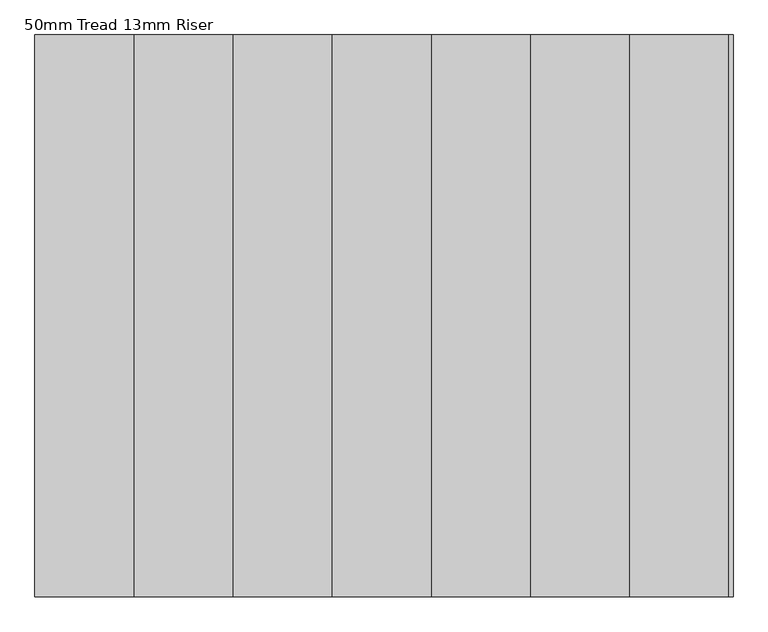
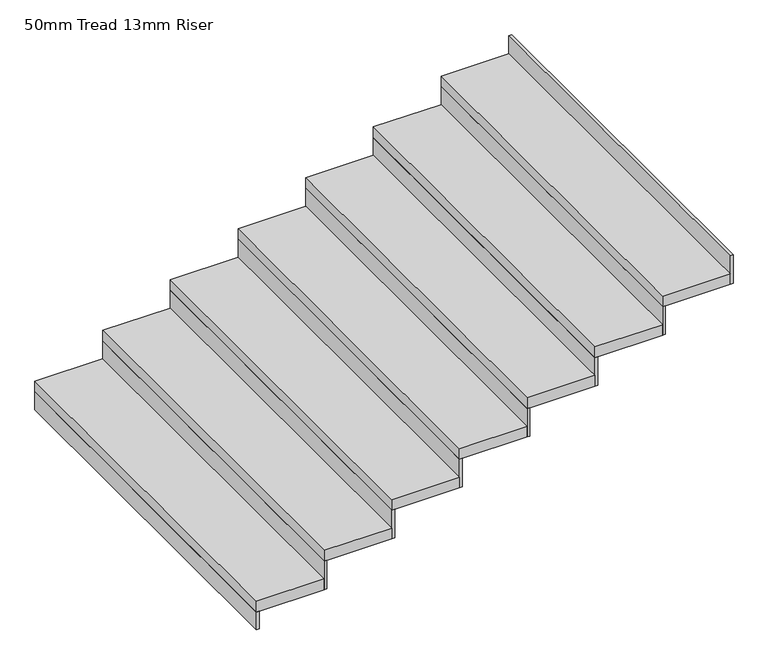
"""IFC4 building model written with IfcOpenShell, lengths in millimetres: stair flight geometry, 50mm Tread 13mm Riser."""

from ifc_helpers import new_model, si_unit, frame, origin, place, context, project, spatial, polyline, outline, extrude, source, transform, mapped, element, save


def stair_flight_50mm_tread_13mm_riser_cbb1d095(model_context):
    return source(origin(), model_context, "Body", "SweptSolid", [
        extrude(outline(polyline([(-15462.7814495, -5518.0731037), (-15475.2814495, -5518.0731037), (-15475.2814495, -3818.0731037), (-15462.7814495, -3818.0731037), (-15462.7814495, -5518.0731037)])), frame((0.0, 0.0, -2133.3333333), z_axis=(0.0, 0.0, 1.0), x_axis=(1.0, 0.0, 0.0)), (0.0, 0.0, 1.0), 83.3333333),
        extrude(outline(polyline([(-15175.2814495, -3818.0731037), (-15175.2814495, -5518.0731037), (-15475.2814495, -5518.0731037), (-15475.2814495, -3818.0731037), (-15175.2814495, -3818.0731037)])), frame((0.0, 0.0, -2050.0), z_axis=(0.0, 0.0, 1.0), x_axis=(1.0, 0.0, 0.0)), (0.0, 0.0, 1.0), 50.0),
        extrude(outline(polyline([(-15162.7814495, -5518.0731037), (-15175.2814495, -5518.0731037), (-15175.2814495, -3818.0731037), (-15162.7814495, -3818.0731037), (-15162.7814495, -5518.0731037)])), frame((0.0, 0.0, -2050.0), z_axis=(0.0, 0.0, 1.0), x_axis=(1.0, 0.0, 0.0)), (0.0, 0.0, 1.0), 133.3333333),
        extrude(outline(polyline([(-14875.2814495, -3818.0731037), (-14875.2814495, -5518.0731037), (-15175.2814495, -5518.0731037), (-15175.2814495, -3818.0731037), (-14875.2814495, -3818.0731037)])), frame((0.0, 0.0, -1916.6666667), z_axis=(0.0, 0.0, 1.0), x_axis=(1.0, 0.0, 0.0)), (0.0, 0.0, 1.0), 50.0),
        extrude(outline(polyline([(-14862.7814495, -5518.0731037), (-14875.2814495, -5518.0731037), (-14875.2814495, -3818.0731037), (-14862.7814495, -3818.0731037), (-14862.7814495, -5518.0731037)])), frame((0.0, 0.0, -1916.6666667), z_axis=(0.0, 0.0, 1.0), x_axis=(1.0, 0.0, 0.0)), (0.0, 0.0, 1.0), 133.3333333),
        extrude(outline(polyline([(-14575.2814495, -3818.0731037), (-14575.2814495, -5518.0731037), (-14875.2814495, -5518.0731037), (-14875.2814495, -3818.0731037), (-14575.2814495, -3818.0731037)])), frame((0.0, 0.0, -1783.3333333), z_axis=(0.0, 0.0, 1.0), x_axis=(1.0, 0.0, 0.0)), (0.0, 0.0, 1.0), 50.0),
        extrude(outline(polyline([(-14562.7814495, -5518.0731037), (-14575.2814495, -5518.0731037), (-14575.2814495, -3818.0731037), (-14562.7814495, -3818.0731037), (-14562.7814495, -5518.0731037)])), frame((0.0, 0.0, -1783.3333333), z_axis=(0.0, 0.0, 1.0), x_axis=(1.0, 0.0, 0.0)), (0.0, 0.0, 1.0), 133.3333333),
        extrude(outline(polyline([(-14275.2814495, -3818.0731037), (-14275.2814495, -5518.0731037), (-14575.2814495, -5518.0731037), (-14575.2814495, -3818.0731037), (-14275.2814495, -3818.0731037)])), frame((0.0, 0.0, -1650.0), z_axis=(0.0, 0.0, 1.0), x_axis=(1.0, 0.0, 0.0)), (0.0, 0.0, 1.0), 50.0),
        extrude(outline(polyline([(-14262.7814495, -5518.0731037), (-14275.2814495, -5518.0731037), (-14275.2814495, -3818.0731037), (-14262.7814495, -3818.0731037), (-14262.7814495, -5518.0731037)])), frame((0.0, 0.0, -1650.0), z_axis=(0.0, 0.0, 1.0), x_axis=(1.0, 0.0, 0.0)), (0.0, 0.0, 1.0), 133.3333333),
        extrude(outline(polyline([(-13975.2814495, -3818.0731037), (-13975.2814495, -5518.0731037), (-14275.2814495, -5518.0731037), (-14275.2814495, -3818.0731037), (-13975.2814495, -3818.0731037)])), frame((0.0, 0.0, -1516.6666667), z_axis=(0.0, 0.0, 1.0), x_axis=(1.0, 0.0, 0.0)), (0.0, 0.0, 1.0), 50.0),
        extrude(outline(polyline([(-13962.7814495, -5518.0731037), (-13975.2814495, -5518.0731037), (-13975.2814495, -3818.0731037), (-13962.7814495, -3818.0731037), (-13962.7814495, -5518.0731037)])), frame((0.0, 0.0, -1516.6666667), z_axis=(0.0, 0.0, 1.0), x_axis=(1.0, 0.0, 0.0)), (0.0, 0.0, 1.0), 133.3333333),
        extrude(outline(polyline([(-13675.2814495, -3818.0731037), (-13675.2814495, -5518.0731037), (-13975.2814495, -5518.0731037), (-13975.2814495, -3818.0731037), (-13675.2814495, -3818.0731037)])), frame((0.0, 0.0, -1383.3333333), z_axis=(0.0, 0.0, 1.0), x_axis=(1.0, 0.0, 0.0)), (0.0, 0.0, 1.0), 50.0),
        extrude(outline(polyline([(-13662.7814495, -5518.0731037), (-13675.2814495, -5518.0731037), (-13675.2814495, -3818.0731037), (-13662.7814495, -3818.0731037), (-13662.7814495, -5518.0731037)])), frame((0.0, 0.0, -1383.3333333), z_axis=(0.0, 0.0, 1.0), x_axis=(1.0, 0.0, 0.0)), (0.0, 0.0, 1.0), 133.3333333),
        extrude(outline(polyline([(-13362.7814495, -5518.0731037), (-13375.2814495, -5518.0731037), (-13375.2814495, -3818.0731037), (-13362.7814495, -3818.0731037), (-13362.7814495, -5518.0731037)])), frame((0.0, 0.0, -1250.0), z_axis=(0.0, 0.0, 1.0), x_axis=(1.0, 0.0, 0.0)), (0.0, 0.0, 1.0), 133.3333333),
        extrude(outline(polyline([(-13375.2814495, -3818.0731037), (-13375.2814495, -5518.0731037), (-13675.2814495, -5518.0731037), (-13675.2814495, -3818.0731037), (-13375.2814495, -3818.0731037)])), frame((0.0, 0.0, -1250.0), z_axis=(0.0, 0.0, 1.0), x_axis=(1.0, 0.0, 0.0)), (0.0, 0.0, 1.0), 50.0),
    ])


if __name__ == "__main__":
    model = new_model("IFC4")
    model_context = context("Model", 3, world=origin())
    ifc_project = project(units=[si_unit("LENGTHUNIT", "METRE", prefix="MILLI")], contexts=[model_context])
    site = spatial("IfcSite", under=ifc_project)
    building = spatial("IfcBuilding", under=site)
    placement = place(None, origin())
    stair_flight_50mm_tread_13mm_riser_shape = stair_flight_50mm_tread_13mm_riser_cbb1d095(model_context)
    element("IfcStairFlight", 1, ObjectType="50mm Tread 13mm Riser", at=placement, inside=building, context=model_context, shape_type="MappedRepresentation", body=[
        mapped(stair_flight_50mm_tread_13mm_riser_shape, transform((0.0, 0.0, 0.0), x_axis=(1.0, 0.0, 0.0), y_axis=(0.0, 1.0, 0.0), z_axis=(0.0, 0.0, 1.0))),
    ])
    save(model, "model.ifc")
